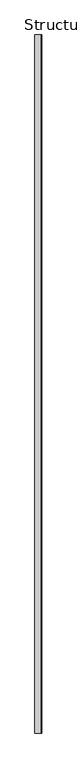
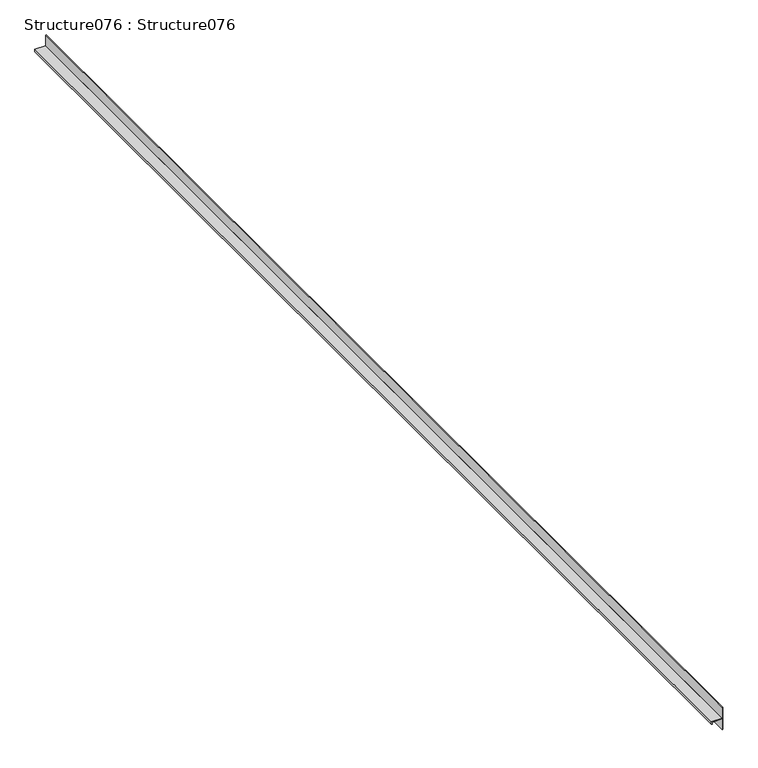
"""IFC4 building model written with IfcOpenShell, lengths in millimetres: proxy geometry, Structure076 : Structure076."""

from ifc_helpers import new_model, si_unit, frame, origin, place, context, project, spatial, polyline, outline, extrude, source, transform, mapped, element, save


def structure076_structure076_2f42f085(model_context):
    return source(origin(), model_context, "Body", "SweptSolid", [
        extrude(outline(polyline([(40144.68, 10020.8312048), (40144.68, 10037.7951528), (40125.63, 10037.7951528), (40125.63, 10039.0651528), (40165.0, 10039.0651528), (40165.0, 10037.7951528), (40145.95, 10037.7951528), (40145.95, 10019.5612048), (40141.2002, 10019.5612048), (40141.2002, 10020.8312048), (40144.68, 10020.8312048)])), frame((0.0, 2217.3609988, 0.0), z_axis=(0.0, 1.0, 0.0), x_axis=(0.0, 0.0, 1.0)), (0.0, 0.0, 1.0), 2000.0),
    ])


if __name__ == "__main__":
    model = new_model("IFC4")
    model_context = context("Model", 3, world=origin())
    ifc_project = project(units=[si_unit("LENGTHUNIT", "METRE", prefix="MILLI")], contexts=[model_context])
    site = spatial("IfcSite", under=ifc_project)
    building = spatial("IfcBuilding", under=site)
    placement = place(None, origin())
    structure076_structure076_shape = structure076_structure076_2f42f085(model_context)
    element("IfcBuildingElementProxy", 1, Name="Structure076 : Structure076", ObjectType="Structure076 : Structure076", at=placement, inside=building, context=model_context, shape_type="MappedRepresentation", body=[
        mapped(structure076_structure076_shape, transform((0.0, 0.0, 0.0), x_axis=(1.0, 0.0, 0.0), y_axis=(0.0, 1.0, 0.0), z_axis=(0.0, 0.0, 1.0))),
    ])
    save(model, "model.ifc")

# Revit data of these elements
# Type "Structure076 : Structure076"
#   NameOverride = "Structure076"
# Element 1 (IfcBuildingElementProxy, "Structure076 : Structure076")
#   Materials on its faces: "16 GA. COPPER VENTED T REVEAL BEAD"
# Materials
#   "16 GA. COPPER VENTED T REVEAL BEAD": class "Unassigned", colour RGB 255 227 10, transparency 0
